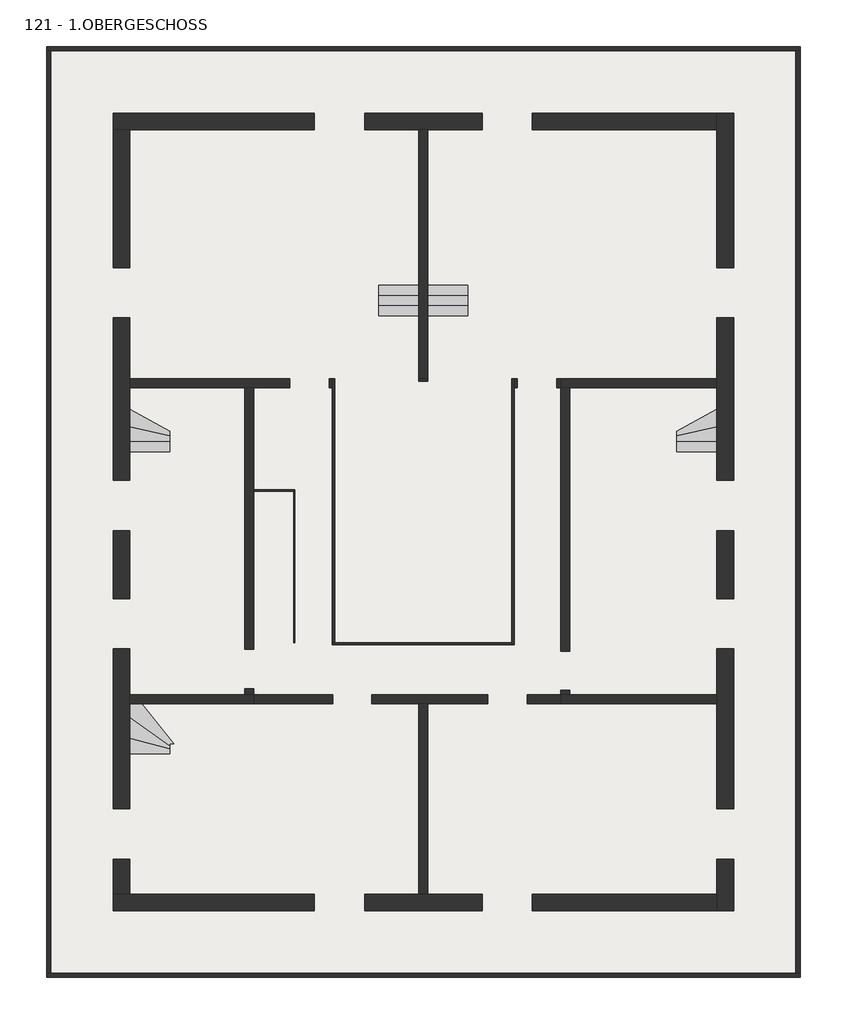
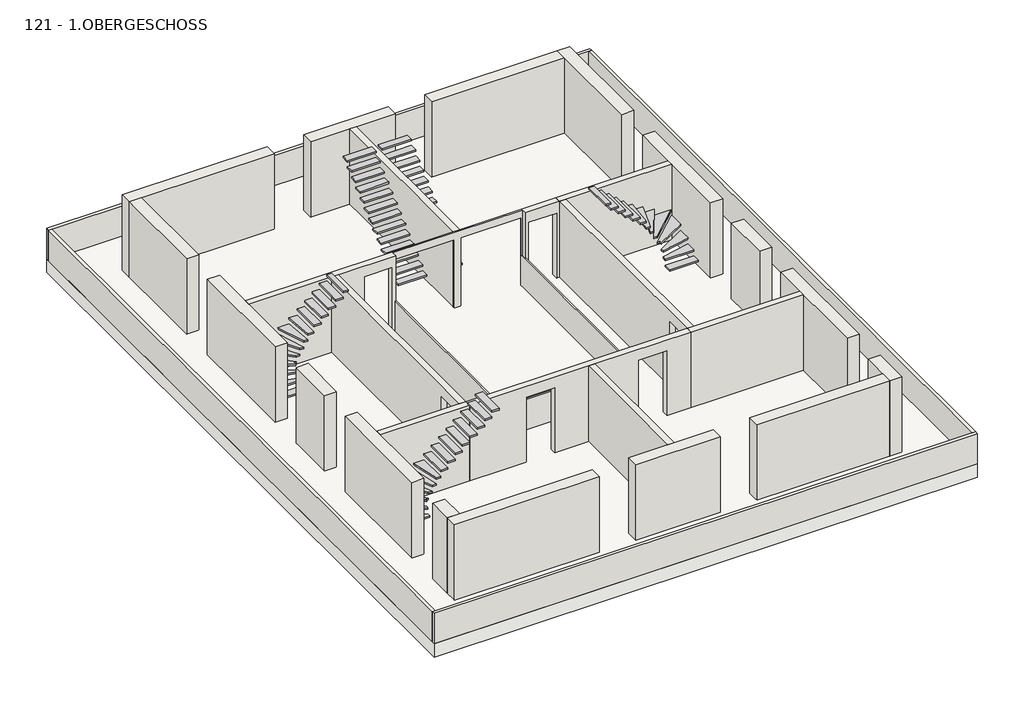
# One storey: 24 walls, 10 stairs, 1 slab.
"""IFC4 building model written with IfcOpenShell, lengths in millimetres."""

import ifcopenshell
import ifcopenshell.guid

model = None  # the IFC model being written
_history = None  # IfcOwnerHistory: only IFC2X3 demands one
_inside = {}  # id of a spatial element -> (the spatial element, [elements in it])
_under = {}  # id of a project, library or spatial element -> (it, [spatial elements below it])
_declared = {}  # id of a project -> (the project, [libraries it declares])
_typed = {}  # id of a type object -> (the type object, [elements of that type])
_made_of = {}  # id of a material, layer set ... -> (it, [elements and type objects made of it])


def new_model(schema):
    """Start an empty IFC model of exactly this schema.

    Asked for "IFC4X3", IfcOpenShell would pick the latest addendum, in which some entities
    have other attributes; the version numbers below select the first issue.
    IFC2X3 requires an IfcOwnerHistory on every rooted entity: one is made here for all.
    """
    global model, _history
    if schema == "IFC4X3":
        model = ifcopenshell.file(schema_version=(4, 3, 0, 0))
    else:
        model = ifcopenshell.file(schema=schema)
    _inside.clear()
    _under.clear()
    _declared.clear()
    _typed.clear()
    _made_of.clear()
    _history = None
    if model.schema == "IFC2X3":
        org = make("IfcOrganization", Name="unknown")
        user = make(
            "IfcPersonAndOrganization",
            ThePerson=make("IfcPerson", FamilyName="unknown"),
            TheOrganization=org,
        )
        app = make(
            "IfcApplication",
            ApplicationDeveloper=org,
            Version="unknown",
            ApplicationFullName="unknown",
            ApplicationIdentifier="unknown",
        )
        _history = make(
            "IfcOwnerHistory",
            OwningUser=user,
            OwningApplication=app,
            ChangeAction="ADDED",
            CreationDate=0,
        )
    return model


def make(cls, **values):
    """One entity of the class cls with the attributes given. An attribute that is None is left unset."""
    return model.create_entity(
        cls, **{name: value for name, value in values.items() if value is not None}
    )


def rooted(cls, **values):
    """An entity with a GlobalId (a new one), such as an element, a storey or a relation."""
    return make(cls, GlobalId=ifcopenshell.guid.new(), OwnerHistory=_history, **values)


def si_unit(unit_type, name, prefix=None):
    """IfcSIUnit, for example si_unit("LENGTHUNIT", "METRE", prefix="MILLI")."""
    return make("IfcSIUnit", UnitType=unit_type, Prefix=prefix, Name=name)


def assignment(units):
    """IfcUnitAssignment: the units of a project."""
    return None if units is None else make("IfcUnitAssignment", Units=units)


def point(xyz):
    """IfcCartesianPoint."""
    return None if xyz is None else make("IfcCartesianPoint", Coordinates=xyz)


def direction(xyz):
    """IfcDirection."""
    return None if xyz is None else make("IfcDirection", DirectionRatios=xyz)


def frame(location, z_axis=None, x_axis=None):
    """IfcAxis2Placement3D, a coordinate frame: its origin and axes. An axis left out is left unset."""
    return make(
        "IfcAxis2Placement3D",
        Location=point(location),
        Axis=direction(z_axis),
        RefDirection=direction(x_axis),
    )


def origin():
    """The frame at (0, 0, 0) with its axes left unset."""
    return frame((0.0, 0.0, 0.0))


def place(relative_to, where):
    """IfcLocalPlacement: puts the frame where relative to a parent placement (None: the world)."""
    return make(
        "IfcLocalPlacement", PlacementRelTo=relative_to, RelativePlacement=where
    )


def context(
    kind, dimensions, precision=None, world=None, true_north=None, identifier=None
):
    """IfcGeometricRepresentationContext, for example the 3D "Model" context."""
    return make(
        "IfcGeometricRepresentationContext",
        ContextIdentifier=identifier,
        ContextType=kind,
        CoordinateSpaceDimension=dimensions,
        Precision=precision,
        WorldCoordinateSystem=world,
        TrueNorth=true_north,
    )


def project(units=None, contexts=None):
    """IfcProject with its units and contexts."""
    return rooted(
        "IfcProject",
        Name="project",
        RepresentationContexts=contexts,
        UnitsInContext=assignment(units),
    )


def spatial(cls, under=None, at=None, **own):
    """A site, building, storey or space (cls), placed at a placement, below another one or the project."""
    s = rooted(cls, ObjectPlacement=at, **own)
    if under is not None:
        _under.setdefault(under.id(), (under, []))[1].append(s)
    return s


def polyline(points):
    """IfcPolyline through the points."""
    return make("IfcPolyline", Points=[point(p) for p in points])


def outline(outer, holes=None, kind="AREA"):
    """IfcArbitraryClosedProfileDef: a profile drawn as a closed curve; with holes, ...WithVoids."""
    if holes is None:
        return make("IfcArbitraryClosedProfileDef", ProfileType=kind, OuterCurve=outer)
    return make(
        "IfcArbitraryProfileDefWithVoids",
        ProfileType=kind,
        OuterCurve=outer,
        InnerCurves=holes,
    )


def extrude(swept, where, along, depth):
    """IfcExtrudedAreaSolid: the profile swept, set in the frame where, extruded along a direction by depth."""
    return make(
        "IfcExtrudedAreaSolid",
        SweptArea=swept,
        Position=where,
        ExtrudedDirection=direction(along),
        Depth=depth,
    )


def faces_of(points, faces, orient=None, outer=None):
    """IfcFace entities. A face is a list of loops; a loop is a list of indices into points, from 0.

    orient and outer hold one flag for each loop. By default every Orientation is true, the
    first loop of a face is its IfcFaceOuterBound and the others are IfcFaceBound.
    """
    made = []
    for i, loops in enumerate(faces):
        bounds = []
        for j, loop in enumerate(loops):
            is_outer = j == 0 if outer is None else outer[i][j]
            bounds.append(
                make(
                    "IfcFaceOuterBound" if is_outer else "IfcFaceBound",
                    Bound=make("IfcPolyLoop", Polygon=[points[k] for k in loop]),
                    Orientation=True if orient is None else orient[i][j],
                )
            )
        made.append(make("IfcFace", Bounds=bounds))
    return made


def faceted_brep(points, faces, orient=None, outer=None, voids=None):
    """IfcFacetedBrep: a solid bounded by flat faces; with voids (closed shells), ...WithVoids."""
    shared = [point(p) for p in points]
    hull = make("IfcClosedShell", CfsFaces=faces_of(shared, faces, orient, outer))
    if voids is None:
        return make("IfcFacetedBrep", Outer=hull)
    return make(
        "IfcFacetedBrepWithVoids",
        Outer=hull,
        Voids=[
            make(cls, CfsFaces=faces_of(shared, fs, o, b)) for cls, fs, o, b in voids
        ],
    )


def shape(context_of_items, identifier, shape_type, items):
    """IfcShapeRepresentation: the items that make up one representation, for example the "Body"."""
    return make(
        "IfcShapeRepresentation",
        ContextOfItems=context_of_items,
        RepresentationIdentifier=identifier,
        RepresentationType=shape_type,
        Items=items,
    )


def source(mapping_origin, context_of_items, identifier, shape_type, items):
    """IfcRepresentationMap: a shape defined once, which mapped items show again and again."""
    return make(
        "IfcRepresentationMap",
        MappingOrigin=mapping_origin,
        MappedRepresentation=shape(context_of_items, identifier, shape_type, items),
    )


def transform(
    local_origin,
    x_axis=None,
    y_axis=None,
    z_axis=None,
    scale=None,
    scale2=None,
    scale3=None,
    uniform=True,
):
    """IfcCartesianTransformationOperator3D, or its non-uniform kind. x_axis, y_axis, z_axis: its Axis1, 2, 3."""
    if uniform:
        return make(
            "IfcCartesianTransformationOperator3D",
            Axis1=direction(x_axis),
            Axis2=direction(y_axis),
            LocalOrigin=point(local_origin),
            Scale=scale,
            Axis3=direction(z_axis),
        )
    return make(
        "IfcCartesianTransformationOperator3DnonUniform",
        Axis1=direction(x_axis),
        Axis2=direction(y_axis),
        LocalOrigin=point(local_origin),
        Scale=scale,
        Axis3=direction(z_axis),
        Scale2=scale2,
        Scale3=scale3,
    )


def mapped(mapping_source, mapping_target):
    """IfcMappedItem: shows the shape of a source again, moved by a transform."""
    return make(
        "IfcMappedItem", MappingSource=mapping_source, MappingTarget=mapping_target
    )


def made_of(thing, what):
    """Note that an element or type object is made of a material, layer set ...; save() writes the relation."""
    if what is not None:
        _made_of.setdefault(what.id(), (what, []))[1].append(thing)
    return thing


def element(
    cls,
    number,
    at=None,
    inside=None,
    cuts=None,
    type_object=None,
    material=None,
    context=None,
    identifier="Body",
    shape_type=None,
    held_by="IfcProductDefinitionShape",
    body=None,
    shapes=None,
    **own,
):
    """One element of the class cls, such as IfcWall. Its Tag is "e" and its number.

    at: its placement. inside: the storey or other place that contains it. cuts: it is an
    opening in that element (IfcRelVoidsElement). A single representation is given by context,
    identifier, shape_type and body (its items); several are given by shapes. held_by: the class
    of the entity that holds the representations. save() writes the other relations.
    """
    e = rooted(cls, Tag="e%d" % number, ObjectPlacement=at, **own)
    if body is not None:
        shapes = [shape(context, identifier, shape_type, body)]
    if shapes is not None:
        e.Representation = make(held_by, Representations=shapes)
    if inside is not None:
        _inside.setdefault(inside.id(), (inside, []))[1].append(e)
    if cuts is not None:
        rooted(
            "IfcRelVoidsElement", RelatingBuildingElement=cuts, RelatedOpeningElement=e
        )
    if type_object is not None:
        _typed.setdefault(type_object.id(), (type_object, []))[1].append(e)
    return made_of(e, material)


def aggregate(whole, parts):
    """IfcRelAggregates: a whole, such as a stair, and the parts it consists of."""
    return rooted("IfcRelAggregates", RelatingObject=whole, RelatedObjects=parts)


def save(model, path):
    """Write the relations noted so far, then the file.

    IfcRelAggregates (storeys below a building ...), IfcRelContainedInSpatialStructure (elements
    in a storey), IfcRelDefinesByType, IfcRelAssociatesMaterial and IfcRelDeclares: one each for
    every whole, place, type object, material and project.
    """
    for whole, parts in _under.values():
        aggregate(whole, parts)
    for where, things in _inside.values():
        rooted(
            "IfcRelContainedInSpatialStructure",
            RelatedElements=things,
            RelatingStructure=where,
        )
    for kind, things in _typed.values():
        rooted("IfcRelDefinesByType", RelatedObjects=things, RelatingType=kind)
    for what, things in _made_of.values():
        rooted("IfcRelAssociatesMaterial", RelatedObjects=things, RelatingMaterial=what)
    for by, libraries in _declared.values():
        rooted("IfcRelDeclares", RelatingContext=by, RelatedDefinitions=libraries)
    model.write(path)


def slab_4f2d1623(model_context):
    return source(origin(), model_context, "Body", "SweptSolid", [
        extrude(outline(polyline([(174297.7593015, 47984.7962965), (174297.7593015, 26981.9343946), (157297.7593015, 26981.9343946), (157297.7593015, 47984.7962965), (174297.7593015, 47984.7962965)])), frame((0.0, 0.0, 2880.0), z_axis=(0.0, 0.0, 1.0), x_axis=(1.0, 0.0, 0.0)), (0.0, 0.0, 1.0), 450.0),
    ])


def stair_92ba3d55(model_context):
    return source(origin(), model_context, "Body", "SweptSolid", [
        extrude(outline(polyline([(160077.7593015, 32139.1812131), (160077.7593015, 32029.7962965), (159177.7593015, 32029.7962965), (159177.7593015, 32381.5903923), (160077.7593015, 32139.1812131)])), frame((0.0, 0.0, 3480.0), z_axis=(0.0, 0.0, 1.0), x_axis=(1.0, 0.0, 0.0)), (0.0, 0.0, 1.0), 50.0),
        extrude(outline(polyline([(160077.7593015, 32208.6851854), (160077.7593015, 32139.1812131), (159177.7593015, 32381.5903923), (159177.7593015, 32851.1265298), (160077.7593015, 32208.6851854)])), frame((0.0, 0.0, 3680.0), z_axis=(0.0, 0.0, 1.0), x_axis=(1.0, 0.0, 0.0)), (0.0, 0.0, 1.0), 50.0),
        extrude(outline(polyline([(159450.38828, 33159.7962965), (160164.4298971, 32259.7962965), (160077.7593015, 32259.7962965), (160077.7593015, 32208.6851854), (159177.7593015, 32851.1265298), (159177.7593015, 33159.7962965), (159450.38828, 33159.7962965)])), frame((0.0, 0.0, 3880.0), z_axis=(0.0, 0.0, 1.0), x_axis=(1.0, 0.0, 0.0)), (0.0, 0.0, 1.0), 50.0),
        extrude(outline(polyline([(160285.4396784, 32259.7962965), (160164.4298971, 32259.7962965), (159450.38828, 33159.7962965), (159877.5404106, 33159.7962965), (160285.4396784, 32259.7962965)])), frame((0.0, 0.0, 4080.0), z_axis=(0.0, 0.0, 1.0), x_axis=(1.0, 0.0, 0.0)), (0.0, 0.0, 1.0), 50.0),
        extrude(outline(polyline([(160412.2916695, 32259.7962965), (160285.4396784, 32259.7962965), (159877.5404106, 33159.7962965), (160212.4306066, 33159.7962965), (160412.2916695, 32259.7962965)])), frame((0.0, 0.0, 4280.0), z_axis=(0.0, 0.0, 1.0), x_axis=(1.0, 0.0, 0.0)), (0.0, 0.0, 1.0), 50.0),
        extrude(outline(polyline([(160546.5910216, 32259.7962965), (160412.2916695, 32259.7962965), (160212.4306066, 33159.7962965), (160538.1312545, 33159.7962965), (160546.5910216, 32259.7962965)])), frame((0.0, 0.0, 4480.0), z_axis=(0.0, 0.0, 1.0), x_axis=(1.0, 0.0, 0.0)), (0.0, 0.0, 1.0), 50.0),
        extrude(outline(polyline([(160772.3611381, 32259.7962965), (160546.5910216, 32259.7962965), (160538.1312545, 33159.7962965), (160772.3611381, 33159.7962965), (160772.3611381, 32259.7962965)])), frame((0.0, 0.0, 4680.0), z_axis=(0.0, 0.0, 1.0), x_axis=(1.0, 0.0, 0.0)), (0.0, 0.0, 1.0), 50.0),
        extrude(outline(polyline([(161002.3611381, 32259.7962965), (160772.3611381, 32259.7962965), (160772.3611381, 33159.7962965), (161002.3611381, 33159.7962965), (161002.3611381, 32259.7962965)])), frame((0.0, 0.0, 4880.0), z_axis=(0.0, 0.0, 1.0), x_axis=(1.0, 0.0, 0.0)), (0.0, 0.0, 1.0), 50.0),
        extrude(outline(polyline([(161232.3611381, 32259.7962965), (161002.3611381, 32259.7962965), (161002.3611381, 33159.7962965), (161232.3611381, 33159.7962965), (161232.3611381, 32259.7962965)])), frame((0.0, 0.0, 5080.0), z_axis=(0.0, 0.0, 1.0), x_axis=(1.0, 0.0, 0.0)), (0.0, 0.0, 1.0), 50.0),
        extrude(outline(polyline([(161462.3611381, 32259.7962965), (161232.3611381, 32259.7962965), (161232.3611381, 33159.7962965), (161462.3611381, 33159.7962965), (161462.3611381, 32259.7962965)])), frame((0.0, 0.0, 5280.0), z_axis=(0.0, 0.0, 1.0), x_axis=(1.0, 0.0, 0.0)), (0.0, 0.0, 1.0), 50.0),
        extrude(outline(polyline([(161692.3611381, 32259.7962965), (161462.3611381, 32259.7962965), (161462.3611381, 33159.7962965), (161692.3611381, 33159.7962965), (161692.3611381, 32259.7962965)])), frame((0.0, 0.0, 5480.0), z_axis=(0.0, 0.0, 1.0), x_axis=(1.0, 0.0, 0.0)), (0.0, 0.0, 1.0), 50.0),
        extrude(outline(polyline([(161922.3611381, 32259.7962965), (161692.3611381, 32259.7962965), (161692.3611381, 33159.7962965), (161922.3611381, 33159.7962965), (161922.3611381, 32259.7962965)])), frame((0.0, 0.0, 5680.0), z_axis=(0.0, 0.0, 1.0), x_axis=(1.0, 0.0, 0.0)), (0.0, 0.0, 1.0), 50.0),
        extrude(outline(polyline([(162152.3611381, 32259.7962965), (161922.3611381, 32259.7962965), (161922.3611381, 33159.7962965), (162152.3611381, 33159.7962965), (162152.3611381, 32259.7962965)])), frame((0.0, 0.0, 5880.0), z_axis=(0.0, 0.0, 1.0), x_axis=(1.0, 0.0, 0.0)), (0.0, 0.0, 1.0), 50.0),
        extrude(outline(polyline([(162382.3611381, 32259.7962965), (162152.3611381, 32259.7962965), (162152.3611381, 33159.7962965), (162382.3611381, 33159.7962965), (162382.3611381, 32259.7962965)])), frame((0.0, 0.0, 6080.0), z_axis=(0.0, 0.0, 1.0), x_axis=(1.0, 0.0, 0.0)), (0.0, 0.0, 1.0), 50.0),
    ])


def stair_5d17669e(model_context):
    return source(origin(), model_context, "Body", "SweptSolid", [
        extrude(outline(polyline([(166797.7593015, 42144.7962965), (166797.7593015, 41914.7962965), (165897.7593015, 41914.7962965), (165897.7593015, 42144.7962965), (166797.7593015, 42144.7962965)])), frame((0.0, 0.0, 3482.1428571), z_axis=(0.0, 0.0, 1.0), x_axis=(1.0, 0.0, 0.0)), (0.0, 0.0, 1.0), 50.0),
        extrude(outline(polyline([(166797.7593015, 42374.7962965), (166797.7593015, 42144.7962965), (165897.7593015, 42144.7962965), (165897.7593015, 42374.7962965), (166797.7593015, 42374.7962965)])), frame((0.0, 0.0, 3684.2857143), z_axis=(0.0, 0.0, 1.0), x_axis=(1.0, 0.0, 0.0)), (0.0, 0.0, 1.0), 50.0),
        extrude(outline(polyline([(166797.7593015, 42604.7962965), (166797.7593015, 42374.7962965), (165897.7593015, 42374.7962965), (165897.7593015, 42604.7962965), (166797.7593015, 42604.7962965)])), frame((0.0, 0.0, 3886.4285714), z_axis=(0.0, 0.0, 1.0), x_axis=(1.0, 0.0, 0.0)), (0.0, 0.0, 1.0), 50.0),
        extrude(outline(polyline([(166797.7593015, 42834.7962965), (166797.7593015, 42604.7962965), (165897.7593015, 42604.7962965), (165897.7593015, 42834.7962965), (166797.7593015, 42834.7962965)])), frame((0.0, 0.0, 4088.5714286), z_axis=(0.0, 0.0, 1.0), x_axis=(1.0, 0.0, 0.0)), (0.0, 0.0, 1.0), 50.0),
        extrude(outline(polyline([(166797.7593015, 43064.7962965), (166797.7593015, 42834.7962965), (165897.7593015, 42834.7962965), (165897.7593015, 43064.7962965), (166797.7593015, 43064.7962965)])), frame((0.0, 0.0, 4290.7142857), z_axis=(0.0, 0.0, 1.0), x_axis=(1.0, 0.0, 0.0)), (0.0, 0.0, 1.0), 50.0),
        extrude(outline(polyline([(166797.7593015, 43294.7962965), (166797.7593015, 43064.7962965), (165897.7593015, 43064.7962965), (165897.7593015, 43294.7962965), (166797.7593015, 43294.7962965)])), frame((0.0, 0.0, 4492.8571429), z_axis=(0.0, 0.0, 1.0), x_axis=(1.0, 0.0, 0.0)), (0.0, 0.0, 1.0), 50.0),
        extrude(outline(polyline([(166797.7593015, 43524.7962965), (166797.7593015, 43294.7962965), (165897.7593015, 43294.7962965), (165897.7593015, 43524.7962965), (166797.7593015, 43524.7962965)])), frame((0.0, 0.0, 4695.0), z_axis=(0.0, 0.0, 1.0), x_axis=(1.0, 0.0, 0.0)), (0.0, 0.0, 1.0), 50.0),
        extrude(outline(polyline([(166797.7593015, 43754.7962965), (166797.7593015, 43524.7962965), (165897.7593015, 43524.7962965), (165897.7593015, 43754.7962965), (166797.7593015, 43754.7962965)])), frame((0.0, 0.0, 4897.1428571), z_axis=(0.0, 0.0, 1.0), x_axis=(1.0, 0.0, 0.0)), (0.0, 0.0, 1.0), 50.0),
        extrude(outline(polyline([(166797.7593015, 43984.7962965), (166797.7593015, 43754.7962965), (165897.7593015, 43754.7962965), (165897.7593015, 43984.7962965), (166797.7593015, 43984.7962965)])), frame((0.0, 0.0, 5099.2857143), z_axis=(0.0, 0.0, 1.0), x_axis=(1.0, 0.0, 0.0)), (0.0, 0.0, 1.0), 50.0),
        extrude(outline(polyline([(166797.7593015, 44214.7962965), (166797.7593015, 43984.7962965), (165897.7593015, 43984.7962965), (165897.7593015, 44214.7962965), (166797.7593015, 44214.7962965)])), frame((0.0, 0.0, 5301.4285714), z_axis=(0.0, 0.0, 1.0), x_axis=(1.0, 0.0, 0.0)), (0.0, 0.0, 1.0), 50.0),
        extrude(outline(polyline([(166797.7593015, 44444.7962965), (166797.7593015, 44214.7962965), (165897.7593015, 44214.7962965), (165897.7593015, 44444.7962965), (166797.7593015, 44444.7962965)])), frame((0.0, 0.0, 5503.5714286), z_axis=(0.0, 0.0, 1.0), x_axis=(1.0, 0.0, 0.0)), (0.0, 0.0, 1.0), 50.0),
        extrude(outline(polyline([(166797.7593015, 44674.7962965), (166797.7593015, 44444.7962965), (165897.7593015, 44444.7962965), (165897.7593015, 44674.7962965), (166797.7593015, 44674.7962965)])), frame((0.0, 0.0, 5705.7142857), z_axis=(0.0, 0.0, 1.0), x_axis=(1.0, 0.0, 0.0)), (0.0, 0.0, 1.0), 50.0),
        extrude(outline(polyline([(166797.7593015, 44904.7962965), (166797.7593015, 44674.7962965), (165897.7593015, 44674.7962965), (165897.7593015, 44904.7962965), (166797.7593015, 44904.7962965)])), frame((0.0, 0.0, 5907.8571429), z_axis=(0.0, 0.0, 1.0), x_axis=(1.0, 0.0, 0.0)), (0.0, 0.0, 1.0), 50.0),
    ])


def stair_42ef58a3(model_context):
    return source(origin(), model_context, "Body", "SweptSolid", [
        extrude(outline(polyline([(165697.7593015, 42144.7962965), (165697.7593015, 41914.7962965), (164797.7593015, 41914.7962965), (164797.7593015, 42144.7962965), (165697.7593015, 42144.7962965)])), frame((0.0, 0.0, 3482.1428571), z_axis=(0.0, 0.0, 1.0), x_axis=(1.0, 0.0, 0.0)), (0.0, 0.0, 1.0), 50.0),
        extrude(outline(polyline([(165697.7593015, 42374.7962965), (165697.7593015, 42144.7962965), (164797.7593015, 42144.7962965), (164797.7593015, 42374.7962965), (165697.7593015, 42374.7962965)])), frame((0.0, 0.0, 3684.2857143), z_axis=(0.0, 0.0, 1.0), x_axis=(1.0, 0.0, 0.0)), (0.0, 0.0, 1.0), 50.0),
        extrude(outline(polyline([(165697.7593015, 42604.7962965), (165697.7593015, 42374.7962965), (164797.7593015, 42374.7962965), (164797.7593015, 42604.7962965), (165697.7593015, 42604.7962965)])), frame((0.0, 0.0, 3886.4285714), z_axis=(0.0, 0.0, 1.0), x_axis=(1.0, 0.0, 0.0)), (0.0, 0.0, 1.0), 50.0),
        extrude(outline(polyline([(165697.7593015, 42834.7962965), (165697.7593015, 42604.7962965), (164797.7593015, 42604.7962965), (164797.7593015, 42834.7962965), (165697.7593015, 42834.7962965)])), frame((0.0, 0.0, 4088.5714286), z_axis=(0.0, 0.0, 1.0), x_axis=(1.0, 0.0, 0.0)), (0.0, 0.0, 1.0), 50.0),
        extrude(outline(polyline([(165697.7593015, 43064.7962965), (165697.7593015, 42834.7962965), (164797.7593015, 42834.7962965), (164797.7593015, 43064.7962965), (165697.7593015, 43064.7962965)])), frame((0.0, 0.0, 4290.7142857), z_axis=(0.0, 0.0, 1.0), x_axis=(1.0, 0.0, 0.0)), (0.0, 0.0, 1.0), 50.0),
        extrude(outline(polyline([(165697.7593015, 43294.7962965), (165697.7593015, 43064.7962965), (164797.7593015, 43064.7962965), (164797.7593015, 43294.7962965), (165697.7593015, 43294.7962965)])), frame((0.0, 0.0, 4492.8571429), z_axis=(0.0, 0.0, 1.0), x_axis=(1.0, 0.0, 0.0)), (0.0, 0.0, 1.0), 50.0),
        extrude(outline(polyline([(165697.7593015, 43524.7962965), (165697.7593015, 43294.7962965), (164797.7593015, 43294.7962965), (164797.7593015, 43524.7962965), (165697.7593015, 43524.7962965)])), frame((0.0, 0.0, 4695.0), z_axis=(0.0, 0.0, 1.0), x_axis=(1.0, 0.0, 0.0)), (0.0, 0.0, 1.0), 50.0),
        extrude(outline(polyline([(165697.7593015, 43754.7962965), (165697.7593015, 43524.7962965), (164797.7593015, 43524.7962965), (164797.7593015, 43754.7962965), (165697.7593015, 43754.7962965)])), frame((0.0, 0.0, 4897.1428571), z_axis=(0.0, 0.0, 1.0), x_axis=(1.0, 0.0, 0.0)), (0.0, 0.0, 1.0), 50.0),
        extrude(outline(polyline([(165697.7593015, 43984.7962965), (165697.7593015, 43754.7962965), (164797.7593015, 43754.7962965), (164797.7593015, 43984.7962965), (165697.7593015, 43984.7962965)])), frame((0.0, 0.0, 5099.2857143), z_axis=(0.0, 0.0, 1.0), x_axis=(1.0, 0.0, 0.0)), (0.0, 0.0, 1.0), 50.0),
        extrude(outline(polyline([(165697.7593015, 44214.7962965), (165697.7593015, 43984.7962965), (164797.7593015, 43984.7962965), (164797.7593015, 44214.7962965), (165697.7593015, 44214.7962965)])), frame((0.0, 0.0, 5301.4285714), z_axis=(0.0, 0.0, 1.0), x_axis=(1.0, 0.0, 0.0)), (0.0, 0.0, 1.0), 50.0),
        extrude(outline(polyline([(165697.7593015, 44444.7962965), (165697.7593015, 44214.7962965), (164797.7593015, 44214.7962965), (164797.7593015, 44444.7962965), (165697.7593015, 44444.7962965)])), frame((0.0, 0.0, 5503.5714286), z_axis=(0.0, 0.0, 1.0), x_axis=(1.0, 0.0, 0.0)), (0.0, 0.0, 1.0), 50.0),
        extrude(outline(polyline([(165697.7593015, 44674.7962965), (165697.7593015, 44444.7962965), (164797.7593015, 44444.7962965), (164797.7593015, 44674.7962965), (165697.7593015, 44674.7962965)])), frame((0.0, 0.0, 5705.7142857), z_axis=(0.0, 0.0, 1.0), x_axis=(1.0, 0.0, 0.0)), (0.0, 0.0, 1.0), 50.0),
        extrude(outline(polyline([(165697.7593015, 44904.7962965), (165697.7593015, 44674.7962965), (164797.7593015, 44674.7962965), (164797.7593015, 44904.7962965), (165697.7593015, 44904.7962965)])), frame((0.0, 0.0, 5907.8571429), z_axis=(0.0, 0.0, 1.0), x_axis=(1.0, 0.0, 0.0)), (0.0, 0.0, 1.0), 50.0),
    ])


def stair_4856ba97(model_context):
    return source(origin(), model_context, "Body", "SweptSolid", [
        extrude(outline(polyline([(159177.7593015, 39074.7962965), (160077.7593015, 39074.7962965), (160077.7593015, 38844.7962965), (159177.7593015, 38844.7962965), (159177.7593015, 39074.7962965)])), frame((0.0, 0.0, 3482.1428571), z_axis=(0.0, 0.0, 1.0), x_axis=(1.0, 0.0, 0.0)), (0.0, 0.0, 1.0), 50.0),
        extrude(outline(polyline([(159177.7593015, 39407.7634868), (160077.7593015, 39201.8291061), (160077.7593015, 39074.7962965), (159177.7593015, 39074.7962965), (159177.7593015, 39407.7634868)])), frame((0.0, 0.0, 3684.2857143), z_axis=(0.0, 0.0, 1.0), x_axis=(1.0, 0.0, 0.0)), (0.0, 0.0, 1.0), 50.0),
        extrude(outline(polyline([(159177.7593015, 39801.0914939), (160077.7593015, 39301.7193734), (160077.7593015, 39201.8291061), (159177.7593015, 39407.7634868), (159177.7593015, 39801.0914939)])), frame((0.0, 0.0, 3886.4285714), z_axis=(0.0, 0.0, 1.0), x_axis=(1.0, 0.0, 0.0)), (0.0, 0.0, 1.0), 50.0),
        extrude(outline(polyline([(159177.7593015, 40284.7962965), (159200.4297176, 40284.7962965), (160147.7593015, 39384.7962965), (160077.7593015, 39384.7962965), (160077.7593015, 39301.7193734), (159177.7593015, 39801.0914939), (159177.7593015, 40284.7962965)])), frame((0.0, 0.0, 4088.5714286), z_axis=(0.0, 0.0, 1.0), x_axis=(1.0, 0.0, 0.0)), (0.0, 0.0, 1.0), 50.0),
        extrude(outline(polyline([(159730.1980238, 40284.7962965), (160258.7713888, 39384.7962965), (160147.7593015, 39384.7962965), (159200.4297176, 40284.7962965), (159730.1980238, 40284.7962965)])), frame((0.0, 0.0, 4290.7142857), z_axis=(0.0, 0.0, 1.0), x_axis=(1.0, 0.0, 0.0)), (0.0, 0.0, 1.0), 50.0),
        extrude(outline(polyline([(160089.4284981, 40284.7962965), (160375.293778, 39384.7962965), (160258.7713888, 39384.7962965), (159730.1980238, 40284.7962965), (160089.4284981, 40284.7962965)])), frame((0.0, 0.0, 4492.8571429), z_axis=(0.0, 0.0, 1.0), x_axis=(1.0, 0.0, 0.0)), (0.0, 0.0, 1.0), 50.0),
        extrude(outline(polyline([(160425.6183342, 40284.7962965), (160499.1039419, 39384.7962965), (160375.293778, 39384.7962965), (160089.4284981, 40284.7962965), (160425.6183342, 40284.7962965)])), frame((0.0, 0.0, 4695.0), z_axis=(0.0, 0.0, 1.0), x_axis=(1.0, 0.0, 0.0)), (0.0, 0.0, 1.0), 50.0),
        extrude(outline(polyline([(160692.3611381, 40284.7962965), (160692.3611381, 39384.7962965), (160499.1039419, 39384.7962965), (160425.6183342, 40284.7962965), (160692.3611381, 40284.7962965)])), frame((0.0, 0.0, 4897.1428571), z_axis=(0.0, 0.0, 1.0), x_axis=(1.0, 0.0, 0.0)), (0.0, 0.0, 1.0), 50.0),
        extrude(outline(polyline([(160922.3611381, 40284.7962965), (160922.3611381, 39384.7962965), (160692.3611381, 39384.7962965), (160692.3611381, 40284.7962965), (160922.3611381, 40284.7962965)])), frame((0.0, 0.0, 5099.2857143), z_axis=(0.0, 0.0, 1.0), x_axis=(1.0, 0.0, 0.0)), (0.0, 0.0, 1.0), 50.0),
        extrude(outline(polyline([(161152.3611381, 40284.7962965), (161152.3611381, 39384.7962965), (160922.3611381, 39384.7962965), (160922.3611381, 40284.7962965), (161152.3611381, 40284.7962965)])), frame((0.0, 0.0, 5301.4285714), z_axis=(0.0, 0.0, 1.0), x_axis=(1.0, 0.0, 0.0)), (0.0, 0.0, 1.0), 50.0),
        extrude(outline(polyline([(161382.3611381, 40284.7962965), (161382.3611381, 39384.7962965), (161152.3611381, 39384.7962965), (161152.3611381, 40284.7962965), (161382.3611381, 40284.7962965)])), frame((0.0, 0.0, 5503.5714286), z_axis=(0.0, 0.0, 1.0), x_axis=(1.0, 0.0, 0.0)), (0.0, 0.0, 1.0), 50.0),
        extrude(outline(polyline([(161612.3611381, 40284.7962965), (161612.3611381, 39384.7962965), (161382.3611381, 39384.7962965), (161382.3611381, 40284.7962965), (161612.3611381, 40284.7962965)])), frame((0.0, 0.0, 5705.7142857), z_axis=(0.0, 0.0, 1.0), x_axis=(1.0, 0.0, 0.0)), (0.0, 0.0, 1.0), 50.0),
        extrude(outline(polyline([(161772.7593015, 40284.7962965), (161772.7593015, 39384.7962965), (161612.3611381, 39384.7962965), (161612.3611381, 40284.7962965), (161772.7593015, 40284.7962965)])), frame((0.0, 0.0, 5907.8571429), z_axis=(0.0, 0.0, 1.0), x_axis=(1.0, 0.0, 0.0)), (0.0, 0.0, 1.0), 50.0),
    ])


def stair_6893023c(model_context):
    return source(origin(), model_context, "Body", "SweptSolid", [
        extrude(outline(polyline([(171517.7593015, 39074.7962965), (172417.7593015, 39074.7962965), (172417.7593015, 38844.7962965), (171517.7593015, 38844.7962965), (171517.7593015, 39074.7962965)])), frame((0.0, 0.0, 3482.1428571), z_axis=(0.0, 0.0, 1.0), x_axis=(1.0, 0.0, 0.0)), (0.0, 0.0, 1.0), 50.0),
        extrude(outline(polyline([(171517.7593015, 39201.8291061), (172417.7593015, 39407.7634868), (172417.7593015, 39074.7962965), (171517.7593015, 39074.7962965), (171517.7593015, 39201.8291061)])), frame((0.0, 0.0, 3684.2857143), z_axis=(0.0, 0.0, 1.0), x_axis=(1.0, 0.0, 0.0)), (0.0, 0.0, 1.0), 50.0),
        extrude(outline(polyline([(171517.7593015, 39301.7193734), (172417.7593015, 39801.0914939), (172417.7593015, 39407.7634868), (171517.7593015, 39201.8291061), (171517.7593015, 39301.7193734)])), frame((0.0, 0.0, 3886.4285714), z_axis=(0.0, 0.0, 1.0), x_axis=(1.0, 0.0, 0.0)), (0.0, 0.0, 1.0), 50.0),
        extrude(outline(polyline([(171517.7593015, 39384.7962965), (171447.7593015, 39384.7962965), (172395.0888853, 40284.7962965), (172417.7593015, 40284.7962965), (172417.7593015, 39801.0914939), (171517.7593015, 39301.7193734), (171517.7593015, 39384.7962965)])), frame((0.0, 0.0, 4088.5714286), z_axis=(0.0, 0.0, 1.0), x_axis=(1.0, 0.0, 0.0)), (0.0, 0.0, 1.0), 50.0),
        extrude(outline(polyline([(171336.7472141, 39384.7962965), (171865.3205791, 40284.7962965), (172395.0888853, 40284.7962965), (171447.7593015, 39384.7962965), (171336.7472141, 39384.7962965)])), frame((0.0, 0.0, 4290.7142857), z_axis=(0.0, 0.0, 1.0), x_axis=(1.0, 0.0, 0.0)), (0.0, 0.0, 1.0), 50.0),
        extrude(outline(polyline([(171220.2248249, 39384.7962965), (171506.0901048, 40284.7962965), (171865.3205791, 40284.7962965), (171336.7472141, 39384.7962965), (171220.2248249, 39384.7962965)])), frame((0.0, 0.0, 4492.8571429), z_axis=(0.0, 0.0, 1.0), x_axis=(1.0, 0.0, 0.0)), (0.0, 0.0, 1.0), 50.0),
        extrude(outline(polyline([(171096.414661, 39384.7962965), (171169.9002687, 40284.7962965), (171506.0901048, 40284.7962965), (171220.2248249, 39384.7962965), (171096.414661, 39384.7962965)])), frame((0.0, 0.0, 4695.0), z_axis=(0.0, 0.0, 1.0), x_axis=(1.0, 0.0, 0.0)), (0.0, 0.0, 1.0), 50.0),
        extrude(outline(polyline([(170903.1574649, 39384.7962965), (170903.1574649, 40284.7962965), (171169.9002687, 40284.7962965), (171096.414661, 39384.7962965), (170903.1574649, 39384.7962965)])), frame((0.0, 0.0, 4897.1428571), z_axis=(0.0, 0.0, 1.0), x_axis=(1.0, 0.0, 0.0)), (0.0, 0.0, 1.0), 50.0),
        extrude(outline(polyline([(170673.1574649, 39384.7962965), (170673.1574649, 40284.7962965), (170903.1574649, 40284.7962965), (170903.1574649, 39384.7962965), (170673.1574649, 39384.7962965)])), frame((0.0, 0.0, 5099.2857143), z_axis=(0.0, 0.0, 1.0), x_axis=(1.0, 0.0, 0.0)), (0.0, 0.0, 1.0), 50.0),
        extrude(outline(polyline([(170443.1574649, 39384.7962965), (170443.1574649, 40284.7962965), (170673.1574649, 40284.7962965), (170673.1574649, 39384.7962965), (170443.1574649, 39384.7962965)])), frame((0.0, 0.0, 5301.4285714), z_axis=(0.0, 0.0, 1.0), x_axis=(1.0, 0.0, 0.0)), (0.0, 0.0, 1.0), 50.0),
        extrude(outline(polyline([(170213.1574649, 39384.7962965), (170213.1574649, 40284.7962965), (170443.1574649, 40284.7962965), (170443.1574649, 39384.7962965), (170213.1574649, 39384.7962965)])), frame((0.0, 0.0, 5503.5714286), z_axis=(0.0, 0.0, 1.0), x_axis=(1.0, 0.0, 0.0)), (0.0, 0.0, 1.0), 50.0),
        extrude(outline(polyline([(169983.1574649, 39384.7962965), (169983.1574649, 40284.7962965), (170213.1574649, 40284.7962965), (170213.1574649, 39384.7962965), (169983.1574649, 39384.7962965)])), frame((0.0, 0.0, 5705.7142857), z_axis=(0.0, 0.0, 1.0), x_axis=(1.0, 0.0, 0.0)), (0.0, 0.0, 1.0), 50.0),
        extrude(outline(polyline([(169822.7593015, 39384.7962965), (169822.7593015, 40284.7962965), (169983.1574649, 40284.7962965), (169983.1574649, 39384.7962965), (169822.7593015, 39384.7962965)])), frame((0.0, 0.0, 5907.8571429), z_axis=(0.0, 0.0, 1.0), x_axis=(1.0, 0.0, 0.0)), (0.0, 0.0, 1.0), 50.0),
    ])


model = new_model("IFC4")

# Units and contexts
model_context = context("Model", 3, world=origin())
ifc_project = project(units=[si_unit("LENGTHUNIT", "METRE", prefix="MILLI")], contexts=[model_context])

# Site, building, storey
site = spatial("IfcSite", under=ifc_project)
building = spatial("IfcBuilding", under=site)
storey = spatial("IfcBuildingStorey", under=building, Name="121 - 1.OBERGESCHOSS", Elevation=2825.0)

# Slab
placement = place(None, origin())
slab_shape = slab_4f2d1623(model_context)
element("IfcSlab", 1, ObjectType="Holzdecke 176 : Holzdecke 176", at=placement, inside=storey, context=model_context, shape_type="MappedRepresentation", body=[
    mapped(slab_shape, transform((-157297.7593015, -26934.7962965, 0.0), x_axis=(1.0, 0.0, 0.0), y_axis=(0.0, 1.0, 0.0), z_axis=(0.0, 0.0, 1.0))),
])

# Stairs
stair_shape = stair_92ba3d55(model_context)
element("IfcStair", 2, ObjectType="  97010 :   97010", at=placement, inside=storey, context=model_context, shape_type="MappedRepresentation", body=[
    mapped(stair_shape, transform((-157297.7593015, -26934.7962965, 0.0), x_axis=(1.0, 0.0, 0.0), y_axis=(0.0, 1.0, 0.0), z_axis=(0.0, 0.0, 1.0))),
])
stair_2_shape = stair_5d17669e(model_context)
element("IfcStair", 3, ObjectType="  97882 :   97882", at=placement, inside=storey, context=model_context, shape_type="MappedRepresentation", body=[
    mapped(stair_2_shape, transform((-157297.7593015, -26934.7962965, 0.0), x_axis=(1.0, 0.0, 0.0), y_axis=(0.0, 1.0, 0.0), z_axis=(0.0, 0.0, 1.0))),
])
stair_3_shape = stair_42ef58a3(model_context)
element("IfcStair", 4, ObjectType="  98300 :   98300", at=placement, inside=storey, context=model_context, shape_type="MappedRepresentation", body=[
    mapped(stair_3_shape, transform((-157297.7593015, -26934.7962965, 0.0), x_axis=(1.0, 0.0, 0.0), y_axis=(0.0, 1.0, 0.0), z_axis=(0.0, 0.0, 1.0))),
])
stair_4_shape = stair_4856ba97(model_context)
element("IfcStair", 5, ObjectType="  98728 :   98728", at=placement, inside=storey, context=model_context, shape_type="MappedRepresentation", body=[
    mapped(stair_4_shape, transform((-157297.7593015, -26934.7962965, 0.0), x_axis=(1.0, 0.0, 0.0), y_axis=(0.0, 1.0, 0.0), z_axis=(0.0, 0.0, 1.0))),
])
stair_5_shape = stair_6893023c(model_context)
element("IfcStair", 6, ObjectType="  99154 :   99154", at=placement, inside=storey, context=model_context, shape_type="MappedRepresentation", body=[
    mapped(stair_5_shape, transform((-157297.7593015, -26934.7962965, 0.0), x_axis=(1.0, 0.0, 0.0), y_axis=(0.0, 1.0, 0.0), z_axis=(0.0, 0.0, 1.0))),
])
element("IfcStair", 7, ObjectType="  149542 :   149542", at=placement, inside=storey, context=model_context, shape_type="MappedRepresentation", body=[
    mapped(stair_shape, transform((-157297.7593015, -26934.7962965, 0.0), x_axis=(1.0, 0.0, 0.0), y_axis=(0.0, 1.0, 0.0), z_axis=(0.0, 0.0, 1.0))),
])
element("IfcStair", 8, ObjectType="  150414 :   150414", at=placement, inside=storey, context=model_context, shape_type="MappedRepresentation", body=[
    mapped(stair_2_shape, transform((-157297.7593015, -26934.7962965, 0.0), x_axis=(1.0, 0.0, 0.0), y_axis=(0.0, 1.0, 0.0), z_axis=(0.0, 0.0, 1.0))),
])
element("IfcStair", 9, ObjectType="  150832 :   150832", at=placement, inside=storey, context=model_context, shape_type="MappedRepresentation", body=[
    mapped(stair_3_shape, transform((-157297.7593015, -26934.7962965, 0.0), x_axis=(1.0, 0.0, 0.0), y_axis=(0.0, 1.0, 0.0), z_axis=(0.0, 0.0, 1.0))),
])
element("IfcStair", 10, ObjectType="  151260 :   151260", at=placement, inside=storey, context=model_context, shape_type="MappedRepresentation", body=[
    mapped(stair_4_shape, transform((-157297.7593015, -26934.7962965, 0.0), x_axis=(1.0, 0.0, 0.0), y_axis=(0.0, 1.0, 0.0), z_axis=(0.0, 0.0, 1.0))),
])
element("IfcStair", 11, ObjectType="  151686 :   151686", at=placement, inside=storey, context=model_context, shape_type="MappedRepresentation", body=[
    mapped(stair_5_shape, transform((-157297.7593015, -26934.7962965, 0.0), x_axis=(1.0, 0.0, 0.0), y_axis=(0.0, 1.0, 0.0), z_axis=(0.0, 0.0, 1.0))),
])

# Walls
element("IfcWall", 12, ObjectType=" :1152", at=placement, inside=storey, context=model_context, shape_type="Brep", body=[
    faceted_brep([(15120.0, 14926.9335014, 5830.0), (15120.0, 14926.9335014, 3330.0), (15120.0, 11259.602585, 3330.0), (15120.0, 11259.602585, 5830.0), (15500.0, 14926.9335014, 3330.0), (15500.0, 14926.9335014, 5830.0), (15500.0, 11259.602585, 5830.0), (15500.0, 11259.602585, 3330.0)], [[[0, 1, 2, 3]], [[4, 5, 6, 7]], [[1, 4, 7, 2]], [[5, 0, 3, 6]], [[1, 0, 5, 4]], [[3, 2, 7, 6]]]),
    faceted_brep([(15120.0, 10124.602585, 5830.0), (15120.0, 10124.602585, 3330.0), (15120.0, 8593.5588642, 3330.0), (15120.0, 8593.5588642, 5830.0), (15500.0, 10124.602585, 3330.0), (15500.0, 10124.602585, 5830.0), (15500.0, 8593.5588642, 5830.0), (15500.0, 8593.5588642, 3330.0)], [[[0, 1, 2, 3]], [[4, 5, 6, 7]], [[1, 4, 7, 2]], [[5, 0, 3, 6]], [[1, 0, 5, 4]], [[3, 2, 7, 6]]]),
    faceted_brep([(15120.0, 7458.5588642, 5830.0), (15120.0, 7458.5588642, 3330.0), (15120.0, 3851.740683, 3330.0), (15120.0, 3851.740683, 5830.0), (15500.0, 7458.5588642, 3330.0), (15500.0, 7458.5588642, 5830.0), (15500.0, 3851.740683, 5830.0), (15500.0, 3851.740683, 3330.0)], [[[0, 1, 2, 3]], [[4, 5, 6, 7]], [[1, 4, 7, 2]], [[5, 0, 3, 6]], [[1, 0, 5, 4]], [[3, 2, 7, 6]]]),
    faceted_brep([(15120.0, 19550.0, 3330.0), (15120.0, 19170.0, 3330.0), (15120.0, 16061.9335014, 3330.0), (15120.0, 16061.9335014, 5830.0), (15120.0, 19170.0, 5830.0), (15120.0, 19550.0, 5830.0), (15500.0, 19550.0, 5830.0), (15500.0, 16061.9335014, 5830.0), (15500.0, 16061.9335014, 3330.0), (15500.0, 19550.0, 3330.0)], [[[0, 1, 2, 3, 4, 5]], [[6, 7, 8, 9]], [[2, 1, 0, 9, 8]], [[5, 4, 3, 7, 6]], [[3, 2, 8, 7]], [[0, 5, 6, 9]]]),
    faceted_brep([(15120.0, 1547.1380981, 3330.0), (15120.0, 1547.1380981, 5830.0), (15120.0, 1927.1380981, 5830.0), (15120.0, 2716.740683, 5830.0), (15120.0, 2716.740683, 3330.0), (15120.0, 1927.1380981, 3330.0), (15500.0, 1547.1380981, 5830.0), (15500.0, 1547.1380981, 3330.0), (15500.0, 2716.740683, 3330.0), (15500.0, 2716.740683, 5830.0)], [[[0, 1, 2, 3, 4, 5]], [[6, 7, 8, 9]], [[7, 0, 5, 4, 8]], [[1, 6, 9, 3, 2]], [[4, 3, 9, 8]], [[1, 0, 7, 6]]]),
])
element("IfcWall", 13, ObjectType=" :1161", at=placement, inside=storey, context=model_context, shape_type="Brep", body=[
    faceted_brep([(15120.0, 1927.1380981, 3330.0), (10960.0, 1927.1380981, 3330.0), (10960.0, 1927.1380981, 5830.0), (15120.0, 1927.1380981, 5830.0), (15120.0, 1547.1380981, 5830.0), (10960.0, 1547.1380981, 5830.0), (10960.0, 1547.1380981, 3330.0), (15120.0, 1547.1380981, 3330.0)], [[[0, 1, 2, 3]], [[4, 5, 6, 7]], [[1, 0, 7, 6]], [[3, 2, 5, 4]], [[2, 1, 6, 5]], [[0, 3, 4, 7]]]),
    faceted_brep([(9825.0, 1927.1380981, 5830.0), (9825.0, 1927.1380981, 3330.0), (7175.0, 1927.1380981, 3330.0), (7175.0, 1927.1380981, 5830.0), (9825.0, 1547.1380981, 3330.0), (9825.0, 1547.1380981, 5830.0), (7175.0, 1547.1380981, 5830.0), (7175.0, 1547.1380981, 3330.0)], [[[0, 1, 2, 3]], [[4, 5, 6, 7]], [[1, 4, 7, 2]], [[5, 0, 3, 6]], [[1, 0, 5, 4]], [[3, 2, 7, 6]]]),
    faceted_brep([(1500.0, 1927.1380981, 3330.0), (1500.0, 1927.1380981, 5830.0), (1880.0, 1927.1380981, 5830.0), (6040.0, 1927.1380981, 5830.0), (6040.0, 1927.1380981, 3330.0), (1880.0, 1927.1380981, 3330.0), (1500.0, 1547.1380981, 5830.0), (1500.0, 1547.1380981, 3330.0), (6040.0, 1547.1380981, 3330.0), (6040.0, 1547.1380981, 5830.0)], [[[0, 1, 2, 3, 4, 5]], [[6, 7, 8, 9]], [[7, 0, 5, 4, 8]], [[1, 6, 9, 3, 2]], [[4, 3, 9, 8]], [[1, 0, 7, 6]]]),
])
element("IfcWall", 14, ObjectType=" :1164", at=placement, inside=storey, context=model_context, shape_type="Brep", body=[
    faceted_brep([(10960.0, 19170.0, 3330.0), (15120.0, 19170.0, 3330.0), (15120.0, 19170.0, 5830.0), (10960.0, 19170.0, 5830.0), (10960.0, 19550.0, 5830.0), (15120.0, 19550.0, 5830.0), (15120.0, 19550.0, 3330.0), (10960.0, 19550.0, 3330.0)], [[[0, 1, 2, 3]], [[4, 5, 6, 7]], [[1, 0, 7, 6]], [[3, 2, 5, 4]], [[0, 3, 4, 7]], [[2, 1, 6, 5]]]),
    faceted_brep([(9825.0, 19170.0, 3330.0), (9825.0, 19170.0, 5830.0), (7175.0, 19170.0, 5830.0), (7175.0, 19170.0, 3330.0), (9825.0, 19550.0, 5830.0), (9825.0, 19550.0, 3330.0), (7175.0, 19550.0, 3330.0), (7175.0, 19550.0, 5830.0)], [[[0, 1, 2, 3]], [[4, 5, 6, 7]], [[5, 0, 3, 6]], [[1, 4, 7, 2]], [[1, 0, 5, 4]], [[3, 2, 7, 6]]]),
    faceted_brep([(1500.0, 19170.0, 5830.0), (1500.0, 19170.0, 3330.0), (1880.0, 19170.0, 3330.0), (6040.0, 19170.0, 3330.0), (6040.0, 19170.0, 5830.0), (1880.0, 19170.0, 5830.0), (1500.0, 19550.0, 3330.0), (1500.0, 19550.0, 5830.0), (6040.0, 19550.0, 5830.0), (6040.0, 19550.0, 3330.0)], [[[0, 1, 2, 3, 4, 5]], [[6, 7, 8, 9]], [[1, 6, 9, 3, 2]], [[7, 0, 5, 4, 8]], [[4, 3, 9, 8]], [[1, 0, 7, 6]]]),
])
element("IfcWall", 15, ObjectType=" :1165", at=placement, inside=storey, context=model_context, shape_type="SweptSolid", body=[
    extrude(outline(polyline([(1880.0, 19170.0), (1880.0, 16061.9335014), (1500.0, 16061.9335014), (1500.0, 19170.0), (1880.0, 19170.0)])), frame((0.0, 0.0, 3330.0), z_axis=(0.0, 0.0, 1.0), x_axis=(1.0, 0.0, 0.0)), (0.0, 0.0, 1.0), 2500.0),
    extrude(outline(polyline([(1500.0, 14926.9335014), (1880.0, 14926.9335014), (1880.0, 11259.602585), (1500.0, 11259.602585), (1500.0, 14926.9335014)])), frame((0.0, 0.0, 3330.0), z_axis=(0.0, 0.0, 1.0), x_axis=(1.0, 0.0, 0.0)), (0.0, 0.0, 1.0), 2500.0),
    extrude(outline(polyline([(1500.0, 10124.602585), (1880.0, 10124.602585), (1880.0, 8593.5588642), (1500.0, 8593.5588642), (1500.0, 10124.602585)])), frame((0.0, 0.0, 3330.0), z_axis=(0.0, 0.0, 1.0), x_axis=(1.0, 0.0, 0.0)), (0.0, 0.0, 1.0), 2500.0),
    extrude(outline(polyline([(1500.0, 7458.5588642), (1880.0, 7458.5588642), (1880.0, 3851.740683), (1500.0, 3851.740683), (1500.0, 7458.5588642)])), frame((0.0, 0.0, 3330.0), z_axis=(0.0, 0.0, 1.0), x_axis=(1.0, 0.0, 0.0)), (0.0, 0.0, 1.0), 2500.0),
    extrude(outline(polyline([(1880.0, 1927.1380981), (1500.0, 1927.1380981), (1500.0, 2716.740683), (1880.0, 2716.740683), (1880.0, 1927.1380981)])), frame((0.0, 0.0, 3330.0), z_axis=(0.0, 0.0, 1.0), x_axis=(1.0, 0.0, 0.0)), (0.0, 0.0, 1.0), 2500.0),
])
element("IfcWall", 16, ObjectType=" :1166", at=placement, inside=storey, context=model_context, shape_type="SweptSolid", body=[
    extrude(outline(polyline([(5830.0, 10525.0), (5830.0, 6475.0), (4330.0, 6475.0), (4330.0, 6500.0), (5590.0, 6500.0), (5590.0, 8400.0), (3330.0, 8400.0), (3330.0, 8600.0), (5590.0, 8600.0), (5590.0, 10500.0), (4330.0, 10500.0), (4330.0, 10525.0), (5830.0, 10525.0)])), frame((0.0, 13500.0, 0.0), z_axis=(0.0, 1.0, 0.0), x_axis=(0.0, 0.0, 1.0)), (0.0, 0.0, 1.0), 50.0),
])
element("IfcWall", 17, ObjectType="Holzwand:1150", at=placement, inside=storey, context=model_context, shape_type="Brep", body=[
    faceted_brep([(11600.0, 13350.0, 3330.0), (11800.0, 13350.0, 3330.0), (15120.0, 13350.0, 3330.0), (15120.0, 13350.0, 5830.0), (11800.0, 13350.0, 5830.0), (11600.0, 13350.0, 5830.0), (11600.0, 13550.0, 3330.0), (11600.0, 13550.0, 5830.0), (15120.0, 13550.0, 5830.0), (15120.0, 13550.0, 3330.0)], [[[0, 1, 2, 3, 4, 5]], [[6, 7, 8, 9]], [[2, 1, 0, 6, 9]], [[5, 4, 3, 8, 7]], [[0, 5, 7, 6]], [[3, 2, 9, 8]]]),
])
element("IfcWall", 18, ObjectType="Holzwand:1151", at=placement, inside=storey, context=model_context, shape_type="Brep", body=[
    faceted_brep([(4675.0, 6425.0, 3330.0), (4475.0, 6425.0, 3330.0), (1880.0, 6425.0, 3330.0), (1880.0, 6425.0, 5830.0), (4475.0, 6425.0, 5830.0), (4675.0, 6425.0, 5830.0), (4675.0, 6225.0, 3330.0), (4675.0, 6225.0, 5830.0), (1880.0, 6225.0, 5830.0), (1880.0, 6225.0, 3330.0)], [[[0, 1, 2, 3, 4, 5]], [[6, 7, 8, 9]], [[2, 1, 0, 6, 9]], [[5, 4, 3, 8, 7]], [[0, 5, 7, 6]], [[3, 2, 9, 8]]]),
])
element("IfcWall", 19, ObjectType="Holzwand:1153", at=placement, inside=storey, context=model_context, shape_type="Brep", body=[
    faceted_brep([(15120.0, 6425.0, 3330.0), (11800.0, 6425.0, 3330.0), (11600.0, 6425.0, 3330.0), (11600.0, 6425.0, 5830.0), (11800.0, 6425.0, 5830.0), (15120.0, 6425.0, 5830.0), (15120.0, 6225.0, 3330.0), (15120.0, 6225.0, 5830.0), (11600.0, 6225.0, 5830.0), (11600.0, 6225.0, 3330.0)], [[[0, 1, 2, 3, 4, 5]], [[6, 7, 8, 9]], [[2, 1, 0, 6, 9]], [[5, 4, 3, 8, 7]], [[3, 2, 9, 8]], [[0, 5, 7, 6]]]),
])
element("IfcWall", 20, ObjectType="Holzwand:1154", at=placement, inside=storey, context=model_context, shape_type="Brep", body=[
    faceted_brep([(5605.0, 11050.0, 3330.0), (4675.0, 11050.0, 3330.0), (4675.0, 11050.0, 4330.0), (5605.0, 11050.0, 4330.0), (5605.0, 11020.0, 3330.0), (5605.0, 11020.0, 4330.0), (5575.0, 11020.0, 4330.0), (4675.0, 11020.0, 4330.0), (4675.0, 11020.0, 3330.0), (5575.0, 11020.0, 3330.0)], [[[0, 1, 2, 3]], [[4, 5, 6, 7, 8, 9]], [[1, 0, 4, 9, 8]], [[3, 2, 7, 6, 5]], [[0, 3, 5, 4]], [[2, 1, 8, 7]]]),
])
element("IfcWall", 21, ObjectType="Holzwand:1155", at=placement, inside=storey, context=model_context, shape_type="SweptSolid", body=[
    extrude(outline(polyline([(5605.0, 11020.0), (5605.0, 7600.0), (5575.0, 7600.0), (5575.0, 11020.0), (5605.0, 11020.0)])), frame((0.0, 0.0, 3330.0), z_axis=(0.0, 0.0, 1.0), x_axis=(1.0, 0.0, 0.0)), (0.0, 0.0, 1.0), 1000.0),
])
element("IfcWall", 22, ObjectType="Holzwand:1156", at=placement, inside=storey, context=model_context, shape_type="SweptSolid", body=[
    extrude(outline(polyline([(6425.0, 5830.0), (13350.0, 5830.0), (13350.0, 3330.0), (7409.5766702, 3330.0), (7409.5766702, 5480.0), (6524.5766702, 5480.0), (6524.5766702, 3330.0), (6425.0, 3330.0), (6425.0, 5830.0)])), frame((11600.0, 0.0, 0.0), z_axis=(1.0, 0.0, 0.0), x_axis=(0.0, 1.0, 0.0)), (0.0, 0.0, 1.0), 200.0),
])
element("IfcWall", 23, ObjectType="Holzwand:1157", at=placement, inside=storey, context=model_context, shape_type="SweptSolid", body=[
    extrude(outline(polyline([(8600.0, 19170.0), (8600.0, 13550.0), (8400.0, 13550.0), (8400.0, 19170.0), (8600.0, 19170.0)])), frame((0.0, 0.0, 3330.0), z_axis=(0.0, 0.0, 1.0), x_axis=(1.0, 0.0, 0.0)), (0.0, 0.0, 1.0), 2500.0),
])
element("IfcWall", 24, ObjectType="Holzwand:1158", at=placement, inside=storey, context=model_context, shape_type="Brep", body=[
    faceted_brep([(4475.0, 6425.0, 5830.0), (4475.0, 13350.0, 5830.0), (4475.0, 13350.0, 3330.0), (4475.0, 7448.3297038, 3330.0), (4475.0, 7448.3297038, 5480.0), (4475.0, 6563.3297038, 5480.0), (4475.0, 6563.3297038, 3330.0), (4475.0, 6425.0, 3330.0), (4675.0, 13350.0, 5830.0), (4675.0, 6425.0, 5830.0), (4675.0, 6425.0, 3330.0), (4675.0, 6563.3297038, 3330.0), (4675.0, 6563.3297038, 5480.0), (4675.0, 7448.3297038, 5480.0), (4675.0, 7448.3297038, 3330.0), (4675.0, 11020.0, 3330.0), (4675.0, 11050.0, 3330.0), (4675.0, 13350.0, 3330.0)], [[[0, 1, 2, 3, 4, 5, 6, 7]], [[8, 9, 10, 11, 12, 13, 14, 15, 16, 17]], [[2, 17, 16, 15, 14, 3]], [[10, 7, 6, 11]], [[1, 0, 9, 8]], [[5, 12, 11, 6]], [[12, 5, 4, 13]], [[13, 4, 3, 14]], [[0, 7, 10, 9]], [[2, 1, 8, 17]]]),
])
element("IfcWall", 25, ObjectType="Holzwand:1159", at=placement, inside=storey, context=model_context, shape_type="Brep", body=[
    faceted_brep([(11600.0, 6225.0, 5830.0), (8600.0, 6225.0, 5830.0), (8400.0, 6225.0, 5830.0), (4675.0, 6225.0, 5830.0), (4675.0, 6225.0, 3330.0), (6455.0, 6225.0, 3330.0), (6455.0, 6225.0, 5480.0), (7340.0, 6225.0, 5480.0), (7340.0, 6225.0, 3330.0), (8400.0, 6225.0, 3330.0), (8600.0, 6225.0, 3330.0), (9960.0, 6225.0, 3330.0), (9960.0, 6225.0, 5480.0), (10845.0, 6225.0, 5480.0), (10845.0, 6225.0, 3330.0), (11600.0, 6225.0, 3330.0), (4675.0, 6425.0, 5830.0), (11600.0, 6425.0, 5830.0), (11600.0, 6425.0, 3330.0), (10845.0, 6425.0, 3330.0), (10845.0, 6425.0, 5480.0), (9960.0, 6425.0, 5480.0), (9960.0, 6425.0, 3330.0), (7340.0, 6425.0, 3330.0), (7340.0, 6425.0, 5480.0), (6455.0, 6425.0, 5480.0), (6455.0, 6425.0, 3330.0), (4675.0, 6425.0, 3330.0)], [[[0, 1, 2, 3, 4, 5, 6, 7, 8, 9, 10, 11, 12, 13, 14, 15]], [[16, 17, 18, 19, 20, 21, 22, 23, 24, 25, 26, 27]], [[15, 14, 19, 18]], [[22, 11, 10, 9, 8, 23]], [[4, 27, 26, 5]], [[3, 2, 1, 0, 17, 16]], [[13, 20, 19, 14]], [[20, 13, 12, 21]], [[21, 12, 11, 22]], [[7, 24, 23, 8]], [[24, 7, 6, 25]], [[25, 6, 5, 26]], [[0, 15, 18, 17]], [[4, 3, 16, 27]]]),
])
element("IfcWall", 26, ObjectType="Holzwand:1160", at=placement, inside=storey, context=model_context, shape_type="SweptSolid", body=[
    extrude(outline(polyline([(8600.0, 6225.0), (8600.0, 1927.1380981), (8400.0, 1927.1380981), (8400.0, 6225.0), (8600.0, 6225.0)])), frame((0.0, 0.0, 3330.0), z_axis=(0.0, 0.0, 1.0), x_axis=(1.0, 0.0, 0.0)), (0.0, 0.0, 1.0), 2500.0),
])
element("IfcWall", 27, ObjectType="Holzwand:1162", at=placement, inside=storey, context=model_context, shape_type="Brep", body=[
    faceted_brep([(6475.0, 13350.0, 5830.0), (4675.0, 13350.0, 5830.0), (4475.0, 13350.0, 5830.0), (1880.0, 13350.0, 5830.0), (1880.0, 13350.0, 3330.0), (4475.0, 13350.0, 3330.0), (4675.0, 13350.0, 3330.0), (5490.0, 13350.0, 3330.0), (5490.0, 13350.0, 5480.0), (6375.0, 13350.0, 5480.0), (6375.0, 13350.0, 3330.0), (6450.0, 13350.0, 3330.0), (6450.0, 13350.0, 4330.0), (6475.0, 13350.0, 4330.0), (1880.0, 13550.0, 5830.0), (6475.0, 13550.0, 5830.0), (6475.0, 13550.0, 4330.0), (6450.0, 13550.0, 4330.0), (6450.0, 13550.0, 3330.0), (6375.0, 13550.0, 3330.0), (6375.0, 13550.0, 5480.0), (5490.0, 13550.0, 5480.0), (5490.0, 13550.0, 3330.0), (1880.0, 13550.0, 3330.0)], [[[0, 1, 2, 3, 4, 5, 6, 7, 8, 9, 10, 11, 12, 13]], [[14, 15, 16, 17, 18, 19, 20, 21, 22, 23]], [[18, 11, 10, 19]], [[4, 23, 22, 7, 6, 5]], [[3, 2, 1, 0, 15, 14]], [[21, 8, 7, 22]], [[8, 21, 20, 9]], [[9, 20, 19, 10]], [[15, 0, 13, 16]], [[16, 13, 12, 17]], [[12, 11, 18, 17]], [[4, 3, 14, 23]]]),
])
element("IfcWall", 28, ObjectType="Holzwand:1163", at=placement, inside=storey, context=model_context, shape_type="SweptSolid", body=[
    extrude(outline(polyline([(5830.0, 11600.0), (5830.0, 10525.0), (4330.0, 10525.0), (4330.0, 10550.0), (3330.0, 10550.0), (3330.0, 10625.0), (5480.0, 10625.0), (5480.0, 11510.0), (3330.0, 11510.0), (3330.0, 11600.0), (5830.0, 11600.0)])), frame((0.0, 13350.0, 0.0), z_axis=(0.0, 1.0, 0.0), x_axis=(0.0, 0.0, 1.0)), (0.0, 0.0, 1.0), 200.0),
])
element("IfcWall", 29, ObjectType=" :1167", at=placement, inside=storey, context=model_context, shape_type="Brep", body=[
    faceted_brep([(10500.0, 13550.0, 3330.0), (10500.0, 7600.0, 3330.0), (10500.0, 7550.0, 3330.0), (10500.0, 7550.0, 4330.0), (10500.0, 7600.0, 4330.0), (10500.0, 13550.0, 4330.0), (10550.0, 13550.0, 3330.0), (10550.0, 13550.0, 4330.0), (10550.0, 7550.0, 4330.0), (10550.0, 7550.0, 3330.0), (10525.0, 13550.0, 4330.0)], [[[0, 1, 2, 3, 4, 5]], [[6, 7, 8, 9]], [[2, 1, 0, 6, 9]], [[5, 4, 3, 8, 7, 10]], [[0, 5, 10, 7, 6]], [[3, 2, 9, 8]]]),
])
element("IfcWall", 30, ObjectType=" :1168", at=placement, inside=storey, context=model_context, shape_type="Brep", body=[
    faceted_brep([(10500.0, 7600.0, 3330.0), (6500.0, 7600.0, 3330.0), (6450.0, 7600.0, 3330.0), (6450.0, 7600.0, 4330.0), (6500.0, 7600.0, 4330.0), (10500.0, 7600.0, 4330.0), (10500.0, 7550.0, 3330.0), (10500.0, 7550.0, 4330.0), (6450.0, 7550.0, 4330.0), (6450.0, 7550.0, 3330.0)], [[[0, 1, 2, 3, 4, 5]], [[6, 7, 8, 9]], [[2, 1, 0, 6, 9]], [[5, 4, 3, 8, 7]], [[3, 2, 9, 8]], [[0, 5, 7, 6]]]),
])
element("IfcWall", 31, ObjectType=" :1169", at=placement, inside=storey, context=model_context, shape_type="Brep", body=[
    faceted_brep([(6500.0, 7600.0, 3330.0), (6500.0, 13550.0, 3330.0), (6500.0, 13550.0, 4330.0), (6500.0, 7600.0, 4330.0), (6450.0, 7600.0, 3330.0), (6450.0, 7600.0, 4330.0), (6450.0, 13550.0, 4330.0), (6450.0, 13550.0, 3330.0), (6475.0, 13550.0, 4330.0)], [[[0, 1, 2, 3]], [[4, 5, 6, 7]], [[1, 0, 4, 7]], [[3, 2, 8, 6, 5]], [[2, 1, 7, 6, 8]], [[0, 3, 5, 4]]]),
])
element("IfcWall", 32, ObjectType="Holzwand:1170", at=placement, inside=storey, context=model_context, shape_type="Brep", body=[
    faceted_brep([(0.0, 20950.0, 3330.0), (100.0, 20950.0, 3330.0), (16900.0, 20950.0, 3330.0), (17000.0, 20950.0, 3330.0), (17000.0, 20950.0, 4330.0), (16900.0, 20950.0, 4330.0), (100.0, 20950.0, 4330.0), (0.0, 20950.0, 4330.0), (0.0, 21050.0, 3330.0), (0.0, 21050.0, 4330.0), (17000.0, 21050.0, 4330.0), (17000.0, 21050.0, 3330.0)], [[[0, 1, 2, 3, 4, 5, 6, 7]], [[8, 9, 10, 11]], [[3, 2, 1, 0, 8, 11]], [[7, 6, 5, 4, 10, 9]], [[0, 7, 9, 8]], [[4, 3, 11, 10]]]),
])
element("IfcWall", 33, ObjectType="Holzwand:1171", at=placement, inside=storey, context=model_context, shape_type="Brep", body=[
    faceted_brep([(17000.0, 147.1380981, 3330.0), (16900.0, 147.1380981, 3330.0), (100.0, 147.1380981, 3330.0), (0.0, 147.1380981, 3330.0), (0.0, 147.1380981, 4330.0), (100.0, 147.1380981, 4330.0), (16900.0, 147.1380981, 4330.0), (17000.0, 147.1380981, 4330.0), (17000.0, 47.1380981, 3330.0), (17000.0, 47.1380981, 4330.0), (0.0, 47.1380981, 4330.0), (0.0, 47.1380981, 3330.0)], [[[0, 1, 2, 3, 4, 5, 6, 7]], [[8, 9, 10, 11]], [[3, 2, 1, 0, 8, 11]], [[7, 6, 5, 4, 10, 9]], [[0, 7, 9, 8]], [[4, 3, 11, 10]]]),
])
element("IfcWall", 34, ObjectType="Holzwand:1172", at=placement, inside=storey, context=model_context, shape_type="SweptSolid", body=[
    extrude(outline(polyline([(16900.0, 147.1380981), (16900.0, 20950.0), (17000.0, 20950.0), (17000.0, 147.1380981), (16900.0, 147.1380981)])), frame((0.0, 0.0, 3330.0), z_axis=(0.0, 0.0, 1.0), x_axis=(1.0, 0.0, 0.0)), (0.0, 0.0, 1.0), 1000.0),
])
element("IfcWall", 35, ObjectType="Holzwand:1173", at=placement, inside=storey, context=model_context, shape_type="SweptSolid", body=[
    extrude(outline(polyline([(100.0, 20950.0), (100.0, 147.1380981), (0.0, 147.1380981), (0.0, 20950.0), (100.0, 20950.0)])), frame((0.0, 0.0, 3330.0), z_axis=(0.0, 0.0, 1.0), x_axis=(1.0, 0.0, 0.0)), (0.0, 0.0, 1.0), 1000.0),
])

save(model, "model.ifc")
